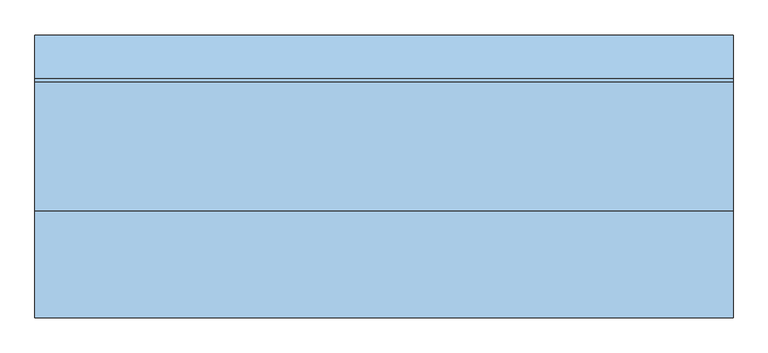
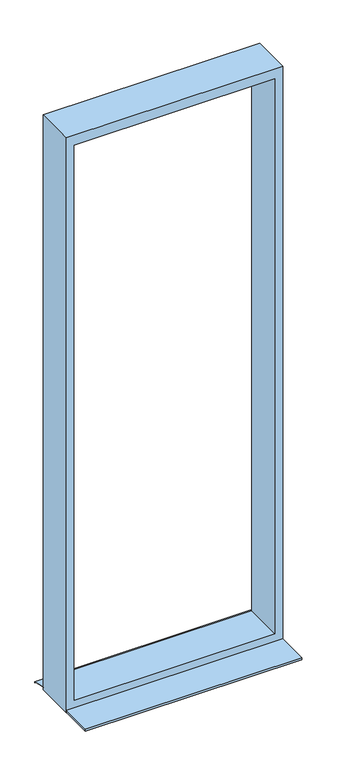
"""IFC4 building model written with IfcOpenShell, lengths in millimetres: window geometry, Fenster - Festverglasung : Feste Verglasung 4.58 x 1.63."""

import ifcopenshell
import ifcopenshell.guid

model = None  # the IFC model being written
_history = None  # IfcOwnerHistory: only IFC2X3 demands one
_inside = {}  # id of a spatial element -> (the spatial element, [elements in it])
_under = {}  # id of a project, library or spatial element -> (it, [spatial elements below it])
_declared = {}  # id of a project -> (the project, [libraries it declares])
_typed = {}  # id of a type object -> (the type object, [elements of that type])
_made_of = {}  # id of a material, layer set ... -> (it, [elements and type objects made of it])


def new_model(schema):
    """Start an empty IFC model of exactly this schema.

    Asked for "IFC4X3", IfcOpenShell would pick the latest addendum, in which some entities
    have other attributes; the version numbers below select the first issue.
    IFC2X3 requires an IfcOwnerHistory on every rooted entity: one is made here for all.
    """
    global model, _history
    if schema == "IFC4X3":
        model = ifcopenshell.file(schema_version=(4, 3, 0, 0))
    else:
        model = ifcopenshell.file(schema=schema)
    _inside.clear()
    _under.clear()
    _declared.clear()
    _typed.clear()
    _made_of.clear()
    _history = None
    if model.schema == "IFC2X3":
        org = make("IfcOrganization", Name="unknown")
        user = make(
            "IfcPersonAndOrganization",
            ThePerson=make("IfcPerson", FamilyName="unknown"),
            TheOrganization=org,
        )
        app = make(
            "IfcApplication",
            ApplicationDeveloper=org,
            Version="unknown",
            ApplicationFullName="unknown",
            ApplicationIdentifier="unknown",
        )
        _history = make(
            "IfcOwnerHistory",
            OwningUser=user,
            OwningApplication=app,
            ChangeAction="ADDED",
            CreationDate=0,
        )
    return model


def make(cls, **values):
    """One entity of the class cls with the attributes given. An attribute that is None is left unset."""
    return model.create_entity(
        cls, **{name: value for name, value in values.items() if value is not None}
    )


def rooted(cls, **values):
    """An entity with a GlobalId (a new one), such as an element, a storey or a relation."""
    return make(cls, GlobalId=ifcopenshell.guid.new(), OwnerHistory=_history, **values)


def si_unit(unit_type, name, prefix=None):
    """IfcSIUnit, for example si_unit("LENGTHUNIT", "METRE", prefix="MILLI")."""
    return make("IfcSIUnit", UnitType=unit_type, Prefix=prefix, Name=name)


def assignment(units):
    """IfcUnitAssignment: the units of a project."""
    return None if units is None else make("IfcUnitAssignment", Units=units)


def point(xyz):
    """IfcCartesianPoint."""
    return None if xyz is None else make("IfcCartesianPoint", Coordinates=xyz)


def direction(xyz):
    """IfcDirection."""
    return None if xyz is None else make("IfcDirection", DirectionRatios=xyz)


def frame(location, z_axis=None, x_axis=None):
    """IfcAxis2Placement3D, a coordinate frame: its origin and axes. An axis left out is left unset."""
    return make(
        "IfcAxis2Placement3D",
        Location=point(location),
        Axis=direction(z_axis),
        RefDirection=direction(x_axis),
    )


def origin():
    """The frame at (0, 0, 0) with its axes left unset."""
    return frame((0.0, 0.0, 0.0))


def place(relative_to, where):
    """IfcLocalPlacement: puts the frame where relative to a parent placement (None: the world)."""
    return make(
        "IfcLocalPlacement", PlacementRelTo=relative_to, RelativePlacement=where
    )


def context(
    kind, dimensions, precision=None, world=None, true_north=None, identifier=None
):
    """IfcGeometricRepresentationContext, for example the 3D "Model" context."""
    return make(
        "IfcGeometricRepresentationContext",
        ContextIdentifier=identifier,
        ContextType=kind,
        CoordinateSpaceDimension=dimensions,
        Precision=precision,
        WorldCoordinateSystem=world,
        TrueNorth=true_north,
    )


def project(units=None, contexts=None):
    """IfcProject with its units and contexts."""
    return rooted(
        "IfcProject",
        Name="project",
        RepresentationContexts=contexts,
        UnitsInContext=assignment(units),
    )


def spatial(cls, under=None, at=None, **own):
    """A site, building, storey or space (cls), placed at a placement, below another one or the project."""
    s = rooted(cls, ObjectPlacement=at, **own)
    if under is not None:
        _under.setdefault(under.id(), (under, []))[1].append(s)
    return s


def polyline(points):
    """IfcPolyline through the points."""
    return make("IfcPolyline", Points=[point(p) for p in points])


def outline(outer, holes=None, kind="AREA"):
    """IfcArbitraryClosedProfileDef: a profile drawn as a closed curve; with holes, ...WithVoids."""
    if holes is None:
        return make("IfcArbitraryClosedProfileDef", ProfileType=kind, OuterCurve=outer)
    return make(
        "IfcArbitraryProfileDefWithVoids",
        ProfileType=kind,
        OuterCurve=outer,
        InnerCurves=holes,
    )


def extrude(swept, where, along, depth):
    """IfcExtrudedAreaSolid: the profile swept, set in the frame where, extruded along a direction by depth."""
    return make(
        "IfcExtrudedAreaSolid",
        SweptArea=swept,
        Position=where,
        ExtrudedDirection=direction(along),
        Depth=depth,
    )


def shape(context_of_items, identifier, shape_type, items):
    """IfcShapeRepresentation: the items that make up one representation, for example the "Body"."""
    return make(
        "IfcShapeRepresentation",
        ContextOfItems=context_of_items,
        RepresentationIdentifier=identifier,
        RepresentationType=shape_type,
        Items=items,
    )


def source(mapping_origin, context_of_items, identifier, shape_type, items):
    """IfcRepresentationMap: a shape defined once, which mapped items show again and again."""
    return make(
        "IfcRepresentationMap",
        MappingOrigin=mapping_origin,
        MappedRepresentation=shape(context_of_items, identifier, shape_type, items),
    )


def transform(
    local_origin,
    x_axis=None,
    y_axis=None,
    z_axis=None,
    scale=None,
    scale2=None,
    scale3=None,
    uniform=True,
):
    """IfcCartesianTransformationOperator3D, or its non-uniform kind. x_axis, y_axis, z_axis: its Axis1, 2, 3."""
    if uniform:
        return make(
            "IfcCartesianTransformationOperator3D",
            Axis1=direction(x_axis),
            Axis2=direction(y_axis),
            LocalOrigin=point(local_origin),
            Scale=scale,
            Axis3=direction(z_axis),
        )
    return make(
        "IfcCartesianTransformationOperator3DnonUniform",
        Axis1=direction(x_axis),
        Axis2=direction(y_axis),
        LocalOrigin=point(local_origin),
        Scale=scale,
        Axis3=direction(z_axis),
        Scale2=scale2,
        Scale3=scale3,
    )


def mapped(mapping_source, mapping_target):
    """IfcMappedItem: shows the shape of a source again, moved by a transform."""
    return make(
        "IfcMappedItem", MappingSource=mapping_source, MappingTarget=mapping_target
    )


def made_of(thing, what):
    """Note that an element or type object is made of a material, layer set ...; save() writes the relation."""
    if what is not None:
        _made_of.setdefault(what.id(), (what, []))[1].append(thing)
    return thing


def element(
    cls,
    number,
    at=None,
    inside=None,
    cuts=None,
    type_object=None,
    material=None,
    context=None,
    identifier="Body",
    shape_type=None,
    held_by="IfcProductDefinitionShape",
    body=None,
    shapes=None,
    **own,
):
    """One element of the class cls, such as IfcWall. Its Tag is "e" and its number.

    at: its placement. inside: the storey or other place that contains it. cuts: it is an
    opening in that element (IfcRelVoidsElement). A single representation is given by context,
    identifier, shape_type and body (its items); several are given by shapes. held_by: the class
    of the entity that holds the representations. save() writes the other relations.
    """
    e = rooted(cls, Tag="e%d" % number, ObjectPlacement=at, **own)
    if body is not None:
        shapes = [shape(context, identifier, shape_type, body)]
    if shapes is not None:
        e.Representation = make(held_by, Representations=shapes)
    if inside is not None:
        _inside.setdefault(inside.id(), (inside, []))[1].append(e)
    if cuts is not None:
        rooted(
            "IfcRelVoidsElement", RelatingBuildingElement=cuts, RelatedOpeningElement=e
        )
    if type_object is not None:
        _typed.setdefault(type_object.id(), (type_object, []))[1].append(e)
    return made_of(e, material)


def aggregate(whole, parts):
    """IfcRelAggregates: a whole, such as a stair, and the parts it consists of."""
    return rooted("IfcRelAggregates", RelatingObject=whole, RelatedObjects=parts)


def save(model, path):
    """Write the relations noted so far, then the file.

    IfcRelAggregates (storeys below a building ...), IfcRelContainedInSpatialStructure (elements
    in a storey), IfcRelDefinesByType, IfcRelAssociatesMaterial and IfcRelDeclares: one each for
    every whole, place, type object, material and project.
    """
    for whole, parts in _under.values():
        aggregate(whole, parts)
    for where, things in _inside.values():
        rooted(
            "IfcRelContainedInSpatialStructure",
            RelatedElements=things,
            RelatingStructure=where,
        )
    for kind, things in _typed.values():
        rooted("IfcRelDefinesByType", RelatedObjects=things, RelatingType=kind)
    for what, things in _made_of.values():
        rooted("IfcRelAssociatesMaterial", RelatedObjects=things, RelatingMaterial=what)
    for by, libraries in _declared.values():
        rooted("IfcRelDeclares", RelatingContext=by, RelatedDefinitions=libraries)
    model.write(path)


def window_80c7f992(model_context):
    return source(origin(), model_context, "Body", "SweptSolid", [
        extrude(outline(polyline([(5580.0, 815.0), (5580.0, -815.0), (1000.0, -815.0), (1000.0, 815.0), (5580.0, 815.0)]), holes=[polyline([(5500.0, 755.0), (1080.0, 755.0), (1080.0, -755.0), (5500.0, -755.0), (5500.0, 755.0)])]), frame((0.0, -80.0, 0.0), z_axis=(0.0, 1.0, 0.0), x_axis=(0.0, 0.0, 1.0)), (0.0, 0.0, 1.0), 300.0),
        extrude(outline(polyline([(-815.0, -330.0), (-815.0, -80.0), (815.0, -80.0), (815.0, -330.0), (-815.0, -330.0)])), frame((0.0, 0.0, 1005.0), z_axis=(0.0, 0.0, 1.0), x_axis=(1.0, 0.0, 0.0)), (0.0, 0.0, 1.0), 15.0),
        extrude(outline(polyline([(230.0221543, 1020.0), (330.0, 1000.0), (330.0, 990.0), (328.0, 990.0), (328.0, 998.3604634), (229.8240723, 1018.0), (220.0, 1018.0), (220.0, 1020.0), (230.0221543, 1020.0)])), frame((-815.0, 0.0, 0.0), z_axis=(1.0, 0.0, 0.0), x_axis=(0.0, 1.0, 0.0)), (0.0, 0.0, 1.0), 1630.0),
    ])


if __name__ == "__main__":
    model = new_model("IFC4")
    model_context = context("Model", 3, world=origin())
    ifc_project = project(units=[si_unit("LENGTHUNIT", "METRE", prefix="MILLI")], contexts=[model_context])
    site = spatial("IfcSite", under=ifc_project)
    building = spatial("IfcBuilding", under=site)
    placement = place(None, origin())
    window_shape = window_80c7f992(model_context)
    element("IfcWindow", 1, ObjectType="Fenster - Festverglasung : Feste Verglasung 4.58 x 1.63", at=placement, inside=building, context=model_context, shape_type="MappedRepresentation", body=[
        mapped(window_shape, transform((0.0, 0.0, 0.0), x_axis=(1.0, 0.0, 0.0), y_axis=(0.0, 1.0, 0.0), z_axis=(0.0, 0.0, 1.0))),
    ])
    save(model, "model.ifc")

# Revit data of these elements
# Type "Fenster - Festverglasung : Feste Verglasung 4.58 x 1.63"
#   Type Mark = "58"
#   Operation = "SinglePanel"
#   Keynote = "16.05.01"
#   Visual Light Transmittance = 0.9
#   Solar Heat Gain Coefficient = 0.78
#   Rough Width = 1.630 m
#   Rough Height = 4.580 m
#   Heat Transfer Coefficient (U) = 3.6886 W/(m²·K)
#   Rahmentiefe = 0.300 m
#   Rahmenhöhe unten = 0.080 m
#   Höhe oberer  Rahmen = 0.080 m
#   Rahmenbreite = 0.060 m
#   Height = 4.580 m
#   Einbautiefe (von außen) [instance default] = 0.080 m
#   Width = 1.630 m
#   Wall Closure = 3
#   Bild [instance default] = none
#   Glas [instance default] = none
#   Innere Fensterbank [instance default] = none
#   Äußere Fensterbank [instance default] = none
#   Construction Type Id = ""
#   Analytic Construction = (empty or 0)
# Element 1 (IfcWindow, "Fenster - Festverglasung : Feste Verglasung 4.58 x 1.63")
#   Materials on its faces: "Kunststoff - Weiß", "Holz - Birke"
# Materials
#   "Kunststoff - Weiß": class "Kunststoff", colour RGB 249 249 249, transparency 0, Cost = 0
#   "Holz - Birke": class "Holz", colour RGB 213 164 103, transparency 0, Cost = 0
